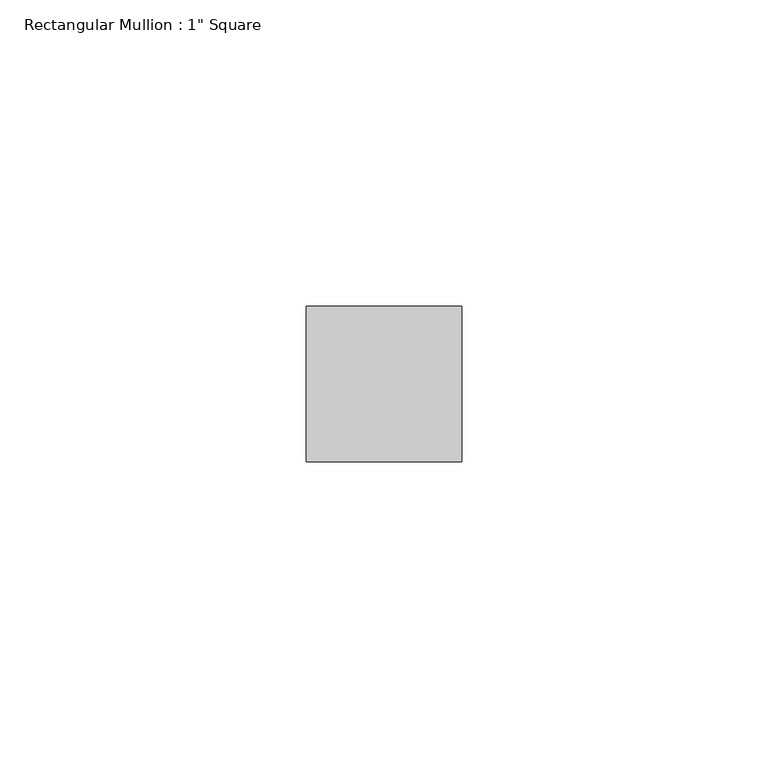
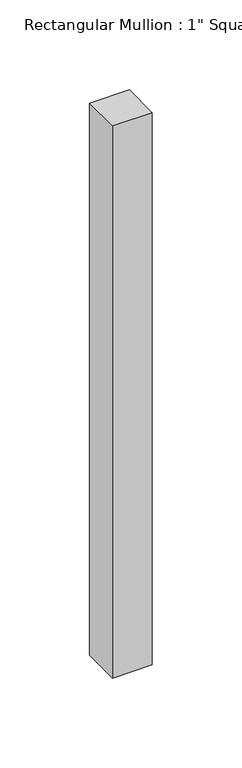
"""IFC4 building model written with IfcOpenShell, lengths in millimetres: member geometry."""

from ifc_helpers import new_model, si_unit, frame, origin, place, context, project, spatial, polyline, outline, extrude, source, transform, mapped, element, save


def member_780c76f3(model_context):
    return source(origin(), model_context, "Body", "SweptSolid", [
        extrude(outline(polyline([(0.0, 12.7), (0.0, -12.7), (-25.4, -12.7), (-25.4, 12.7), (0.0, 12.7)])), frame((0.0, 0.0, -374.6499997), z_axis=(0.0, 0.0, 1.0), x_axis=(1.0, 0.0, 0.0)), (0.0, 0.0, 1.0), 374.6499997),
    ])


if __name__ == "__main__":
    model = new_model("IFC4")
    model_context = context("Model", 3, world=origin())
    ifc_project = project(units=[si_unit("LENGTHUNIT", "METRE", prefix="MILLI")], contexts=[model_context])
    site = spatial("IfcSite", under=ifc_project)
    building = spatial("IfcBuilding", under=site)
    placement = place(None, origin())
    member_shape = member_780c76f3(model_context)
    element("IfcMember", 1, ObjectType="Rectangular Mullion : 1\" Square", at=placement, inside=building, context=model_context, shape_type="MappedRepresentation", body=[
        mapped(member_shape, transform((0.0, 0.0, 0.0), x_axis=(1.0, 0.0, 0.0), y_axis=(0.0, 1.0, 0.0), z_axis=(0.0, 0.0, 1.0))),
    ])
    save(model, "model.ifc")

# Revit data of these elements
# Type "Rectangular Mullion : 1\" Square"
#   built-in parameter 1007304 = 0.0833333 (stored number, unit not read)
#   built-in parameter 1007301 = 0.0416667 (stored number, unit not read)
#   built-in parameter 1007300 = 0.0416667 (stored number, unit not read)
# Element 1 (IfcMember, "Rectangular Mullion : 1\" Square")
#   Materials on its faces: "Metal - Aluminum"
# Materials
#   "Metal - Aluminum": class "Metal", colour RGB 247 247 247, transparency 0
